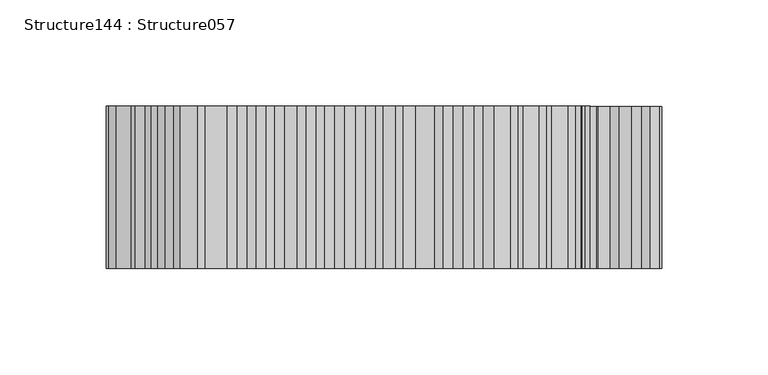
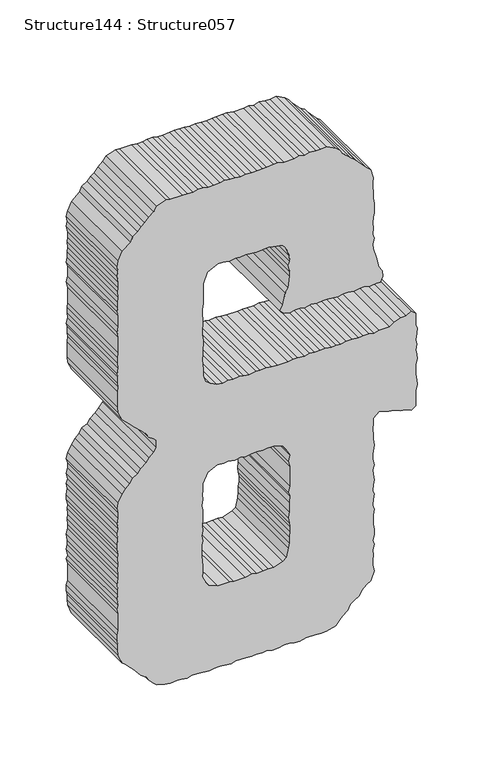
"""IFC4 building model written with IfcOpenShell, lengths in millimetres: proxy geometry, Structure144 : Structure057."""

from ifc_helpers import new_model, si_unit, frame, origin, place, context, project, spatial, polyline, outline, extrude, source, transform, mapped, element, save


def structure144_structure057_dd4a27d7(model_context):
    return source(origin(), model_context, "Body", "SweptSolid", [
        extrude(outline(polyline([(3904.3901392, -40802.0153959), (3895.0048075, -40802.0153959), (3890.320967, -40803.1963849), (3885.0626781, -40802.0153959), (3870.9790644, -40802.0153959), (3866.8776953, -40802.6171226), (3861.6178018, -40802.6171226), (3856.9179152, -40802.0153959), (3852.2340747, -40803.1963849), (3849.3008577, -40802.6171226), (3843.432819, -40802.6171226), (3839.9331766, -40802.0153959), (3835.2332901, -40802.6171226), (3821.1737455, -40802.6171226), (3815.9154565, -40802.0153959), (3808.290376, -40798.4948937), (3804.7730829, -40794.9952513), (3802.448011, -40792.6332735), (3798.3305959, -40788.5543688), (3791.8865042, -40781.5117597), (3787.7867397, -40777.9912574), (3784.2614236, -40775.6517441), (3781.3282066, -40771.550375), (3779.0031347, -40769.2108616), (3772.5606477, -40769.2108616), (3769.0176809, -40771.550375), (3764.9435901, -40775.0500174), (3761.418274, -40777.9912574), (3757.8753073, -40782.6718888), (3753.8012165, -40785.0338666), (3751.4424479, -40789.7128933), (3747.3587295, -40792.0540112), (3743.8414364, -40795.5745135), (3739.7416719, -40798.4948937), (3733.2991849, -40802.0153959), (3728.0152223, -40803.1963849), (3723.9154578, -40802.0153959), (3719.2316172, -40802.0153959), (3714.5301261, -40803.1963849), (3709.2718371, -40802.0153959), (3705.1720727, -40803.1963849), (3700.4705815, -40802.6171226), (3694.6298211, -40803.1963849), (3690.512406, -40803.1963849), (3685.8285655, -40802.0153959), (3682.3289231, -40802.6171226), (3676.4432338, -40802.0153959), (3672.3691429, -40802.6171226), (3667.0851803, -40802.0153959), (3663.5598643, -40802.0153959), (3658.8840468, -40803.1963849), (3652.9999621, -40802.6171226), (3648.9258713, -40802.6171226), (3644.8245022, -40803.1963849), (3638.9580681, -40802.0153959), (3636.0408972, -40803.1963849), (3631.3410106, -40802.0153959), (3616.0972679, -40802.0153959), (3612.0135494, -40803.1963849), (3606.7295868, -40803.1963849), (3603.2122938, -40802.6171226), (3597.9540049, -40802.6171226), (3593.2541183, -40802.0153959), (3585.0706354, -40799.0741559), (3582.7102621, -40796.1762402), (3578.0103756, -40791.474749), (3575.6853037, -40789.1336311), (3570.9854171, -40785.0338666), (3568.0682461, -40782.6718888), (3564.54293, -40777.9912574), (3561.6257591, -40776.2310063), (3557.5003209, -40772.1296372), (3554.5831499, -40768.609135), (3552.242032, -40761.5889903), (3551.6675836, -40756.908359), (3552.242032, -40751.0467387), (3552.242032, -40747.5262365), (3551.0658569, -40742.2663429), (3552.242032, -40738.144114), (3552.242032, -40732.2824938), (3551.0658569, -40722.9003713), (3552.242032, -40718.8214667), (3552.242032, -40714.1408353), (3551.6675836, -40710.0186064), (3551.0658569, -40704.1794506), (3552.242032, -40700.0556171), (3552.242032, -40691.2752213), (3551.6675836, -40685.9944679), (3552.242032, -40682.4948255), (3551.6675836, -40677.2349319), (3552.242032, -40672.5334408), (3551.0658569, -40668.4320717), (3551.0658569, -40662.547987), (3552.242032, -40657.8689603), (3552.242032, -40653.7900557), (3551.0658569, -40649.0885645), (3551.0658569, -40644.4079332), (3552.242032, -40639.1480396), (3552.242032, -40630.9244416), (3551.6675836, -40625.6420836), (3552.242032, -40621.5647836), (3554.0087015, -40613.3411855), (3558.684519, -40609.8415431), (3561.025637, -40607.5020298), (3564.54293, -40602.798934), (3569.2524442, -40600.4594206), (3571.5678885, -40597.5181806), (3574.5107332, -40592.8375493), (3578.6104977, -40590.4980359), (3582.7102621, -40586.3966668), (3585.0706354, -40582.8761646), (3593.2541183, -40579.9333199), (3598.5284533, -40581.1143088), (3602.6298224, -40581.1143088), (3607.8961343, -40580.5350466), (3612.5976255, -40581.1143088), (3617.2718384, -40579.9333199), (3621.3732075, -40581.1143088), (3626.0554434, -40579.9333199), (3631.3410106, -40579.9333199), (3636.0408972, -40580.5350466), (3644.2420307, -40580.5350466), (3649.5003197, -40579.9333199), (3653.6000842, -40581.1143088), (3658.8840468, -40580.5350466), (3663.5598643, -40579.9333199), (3667.0851803, -40581.1143088), (3672.3691429, -40580.5350466), (3676.4432338, -40579.9333199), (3682.3289231, -40580.5350466), (3686.4030139, -40581.1143088), (3690.512406, -40579.9333199), (3695.786741, -40581.1143088), (3700.4705815, -40581.1143088), (3708.6717151, -40579.9333199), (3713.9556777, -40580.5350466), (3718.0554422, -40580.5350466), (3723.9154578, -40581.1143088), (3728.5992983, -40580.5350466), (3733.2991849, -40580.5350466), (3737.9750024, -40575.2542932), (3735.0578314, -40567.0531596), (3734.47536, -40562.3725283), (3732.1149867, -40557.1126348), (3731.5325153, -40552.4111436), (3729.1737467, -40547.7305123), (3732.1149867, -40543.6291432), (3745.6000829, -40543.6291432), (3751.4424479, -40542.4706188), (3755.559863, -40543.0274165), (3760.818152, -40543.6291432), (3770.2018791, -40543.6291432), (3774.8857196, -40542.4706188), (3779.5872107, -40543.0274165), (3783.0868532, -40543.6291432), (3788.3611881, -40543.0274165), (3792.4705802, -40543.6291432), (3798.3305959, -40543.0274165), (3803.0064134, -40542.4706188), (3806.5317294, -40543.6291432), (3817.090027, -40543.6291432), (3820.015221, -40547.7305123), (3817.6741031, -40551.8302768), (3817.090027, -40556.5333726), (3815.3313805, -40562.3725283), (3812.3901405, -40566.4722928), (3812.3901405, -40575.2542932), (3811.2043377, -40579.9333199), (3812.3901405, -40584.0571535), (3812.3901405, -40589.317047), (3811.7884138, -40593.439276), (3812.3901405, -40598.6991695), (3812.3901405, -40603.9799229), (3811.2043377, -40608.6605542), (3811.7884138, -40612.7619233), (3811.2043377, -40616.8841523), (3812.3901405, -40622.1440458), (3811.7884138, -40626.8246771), (3811.7884138, -40631.5261683), (3812.3901405, -40635.6050729), (3811.2043377, -40640.2840996), (3811.7884138, -40646.1681843), (3811.7884138, -40650.2695534), (3811.2043377, -40654.3693179), (3811.2043377, -40663.7305805), (3811.7884138, -40669.0113339), (3812.3901405, -40673.6919652), (3811.7884138, -40678.9743232), (3812.3901405, -40682.4948255), (3811.2043377, -40688.3564457), (3811.7884138, -40693.0354724), (3812.3901405, -40696.5575793), (3811.7884138, -40702.4191995), (3812.3901405, -40706.518964), (3811.2043377, -40711.1995953), (3812.3901405, -40716.4594888), (3815.3313805, -40722.3419689), (3818.2309008, -40726.443338), (3824.1149855, -40728.2035891), (3829.9733965, -40728.2035891), (3839.3587282, -40729.3621136), (3843.432819, -40728.7828514), (3848.7167816, -40728.7828514), (3852.8181507, -40728.2035891), (3856.9179152, -40728.2035891), (3862.8036045, -40729.3621136), (3866.8776953, -40729.3621136), (3871.5599312, -40728.7828514), (3876.263027, -40728.7828514), (3880.9452629, -40729.3621136), (3885.0626781, -40729.3621136), (3890.905043, -40728.2035891), (3908.46423, -40728.2035891), (3917.8479571, -40724.6830869), (3922.5494483, -40715.8802266), (3922.5494483, -40711.1995953), (3921.3748778, -40705.9397018), (3922.5494483, -40700.6364839), (3921.9733953, -40696.5575793), (3922.5494483, -40691.876948), (3921.9733953, -40685.9944679), (3921.3748778, -40682.4948255), (3921.9733953, -40677.2349319), (3922.5494483, -40671.9317141), (3921.3748778, -40667.8528095), (3919.6066036, -40659.0499492), (3916.6653636, -40656.7104358), (3908.46423, -40653.7900557), (3903.2059411, -40653.188329), (3899.7046941, -40654.3693179), (3893.246161, -40653.188329), (3889.1463965, -40653.188329), (3879.1769888, -40654.3693179), (3875.686974, -40657.2896981), (3865.1190488, -40659.0499492), (3860.4432313, -40661.9911892), (3856.9179152, -40657.8689603), (3855.7353217, -40653.188329), (3856.9179152, -40648.5076977), (3856.9179152, -40644.4079332), (3855.7353217, -40640.2840996), (3856.9179152, -40635.0258107), (3856.3161885, -40629.7659172), (3856.9179152, -40625.0628214), (3856.9179152, -40620.9630569), (3855.7353217, -40611.5809344), (3856.9179152, -40606.9003031), (3856.9179152, -40602.798934), (3855.7353217, -40597.5181806), (3856.9179152, -40593.439276), (3856.9179152, -40588.7361802), (3855.7353217, -40583.4778913), (3856.3161885, -40578.1955333), (3856.3161885, -40574.675031), (3861.0192843, -40572.3563775), (3866.3032469, -40572.9131753), (3870.9790644, -40575.8560199), (3880.3627915, -40578.1955333), (3889.1463965, -40580.5350466), (3893.246161, -40581.1143088), (3898.5301236, -40579.9333199), (3902.6314927, -40581.1143088), (3908.46423, -40580.5350466), (3913.1641166, -40581.1143088), (3917.8479571, -40580.5350466), (3921.3748778, -40579.9333199), (3930.7329312, -40579.9333199), (3935.4328178, -40580.5350466), (3940.718385, -40580.5350466), (3945.9766739, -40581.1143088), (3950.0940891, -40581.1143088), (3954.1778075, -40580.5350466), (3962.3757319, -40582.8761646), (3965.3201811, -40586.3966668), (3973.5197101, -40594.0185382), (3976.4368811, -40596.3580516), (3978.8036727, -40599.8801584), (3986.4046842, -40607.5020298), (3989.9460463, -40609.8415431), (3992.8375436, -40613.3411855), (3996.9645864, -40620.9630569), (3996.390138, -40626.2438103), (3996.390138, -40630.3451794), (3996.9645864, -40635.6050729), (3995.7803883, -40640.2840996), (3996.9645864, -40644.9871954), (3995.7803883, -40649.0885645), (3995.7803883, -40657.8689603), (3996.9645864, -40663.7305805), (3996.9645864, -40667.2510828), (3996.390138, -40673.112703), (3996.390138, -40676.6332053), (3995.7803883, -40681.3138366), (3995.7803883, -40685.9944679), (3996.390138, -40691.2752213), (3995.7803883, -40695.9558526), (3996.390138, -40700.6364839), (3996.390138, -40704.7587129), (3996.9645864, -40709.4393442), (3996.390138, -40713.5615731), (3995.7803883, -40719.4007289), (3995.7803883, -40724.0813602), (3996.9645864, -40728.2035891), (3996.9645864, -40732.8842205), (3995.7803883, -40736.9839849), (3995.7803883, -40741.6646163), (3996.390138, -40746.3452476), (3996.390138, -40756.908359), (3996.9645864, -40760.4080014), (3994.0233463, -40768.609135), (3989.9460463, -40771.550375), (3986.4046842, -40775.6517441), (3982.3225704, -40779.1722463), (3979.9621971, -40782.1134864), (3976.4368811, -40785.0338666), (3973.5197101, -40789.7128933), (3968.8198235, -40791.474749), (3962.9774586, -40798.4948937), (3955.360401, -40802.0153959), (3950.6765605, -40803.1963849), (3945.9766739, -40802.6171226), (3941.2912288, -40803.1963849), (3936.0345445, -40802.0153959), (3930.7329312, -40802.0153959), (3927.2332888, -40802.6171226), (3921.9733953, -40802.0153959), (3917.8479571, -40802.6171226), (3912.5896682, -40802.6171226), (3908.46423, -40803.1963849), (3904.3901392, -40802.0153959)]), holes=[polyline([(3735.0578314, -40659.0499492), (3731.5325153, -40656.7104358), (3725.0996559, -40653.188329), (3719.8140887, -40654.3693179), (3714.5301261, -40653.188329), (3696.9709391, -40653.188329), (3691.0868544, -40654.3693179), (3687.587212, -40653.188329), (3681.7271964, -40653.7900557), (3672.9435914, -40653.7900557), (3667.6853024, -40654.3693179), (3662.9854159, -40653.7900557), (3659.4584952, -40653.188329), (3654.7842823, -40653.188329), (3650.1004418, -40653.7900557), (3644.8245022, -40653.7900557), (3640.114988, -40654.3693179), (3631.915459, -40656.1087092), (3629.5984101, -40659.0499492), (3626.6571701, -40667.2510828), (3627.2396415, -40671.9317141), (3626.6571701, -40676.053943), (3626.6571701, -40681.9155633), (3627.2396415, -40685.9944679), (3626.0554434, -40691.876948), (3626.0554434, -40701.8174728), (3626.6571701, -40705.3379751), (3626.6571701, -40715.8802266), (3630.1824862, -40723.502098), (3632.5155811, -40725.2623491), (3639.5405396, -40728.7828514), (3644.2420307, -40728.2035891), (3649.5003197, -40728.2035891), (3658.8840468, -40729.3621136), (3668.8261762, -40729.3621136), (3672.3691429, -40728.2035891), (3677.6274319, -40729.3621136), (3681.7271964, -40728.2035891), (3687.0127636, -40728.7828514), (3691.6869765, -40728.2035891), (3700.4705815, -40728.2035891), (3705.1720727, -40729.3621136), (3710.4560353, -40728.2035891), (3715.1302482, -40728.7828514), (3719.2316172, -40728.2035891), (3725.0996559, -40728.2035891), (3733.8736333, -40724.0813602), (3737.9750024, -40715.8802266), (3737.400554, -40710.0186064), (3737.9750024, -40706.518964), (3736.7988273, -40700.6364839), (3737.9750024, -40695.9558526), (3736.7988273, -40691.2752213), (3737.400554, -40687.1754568), (3737.9750024, -40681.9155633), (3737.400554, -40676.053943), (3737.9750024, -40672.5334408), (3737.9750024, -40667.2510828), (3735.0578314, -40659.0499492)])]), frame((0.0, 247945.1599557, 0.0), z_axis=(0.0, 1.0, 0.0), x_axis=(0.0, 0.0, 1.0)), (0.0, 0.0, 1.0), 76.2),
    ])


if __name__ == "__main__":
    model = new_model("IFC4")
    model_context = context("Model", 3, world=origin())
    ifc_project = project(units=[si_unit("LENGTHUNIT", "METRE", prefix="MILLI")], contexts=[model_context])
    site = spatial("IfcSite", under=ifc_project)
    building = spatial("IfcBuilding", under=site)
    placement = place(None, origin())
    structure144_structure057_shape = structure144_structure057_dd4a27d7(model_context)
    element("IfcBuildingElementProxy", 1, Name="Structure144 : Structure057", ObjectType="Structure144 : Structure057", at=placement, inside=building, context=model_context, shape_type="MappedRepresentation", body=[
        mapped(structure144_structure057_shape, transform((0.0, 0.0, 0.0), x_axis=(1.0, 0.0, 0.0), y_axis=(0.0, 1.0, 0.0), z_axis=(0.0, 0.0, 1.0))),
    ])
    save(model, "model.ifc")

# Revit data of these elements
# Type "Structure144 : Structure057"
#   NameOverride = "Structure057"
# Element 1 (IfcBuildingElementProxy, "Structure144 : Structure057")
#   Materials on its faces: "BRUSHED ALUM. LETTERING"
# Materials
#   "BRUSHED ALUM. LETTERING": class "Unassigned", colour RGB 169 181 186, transparency 0, Cost = 0
